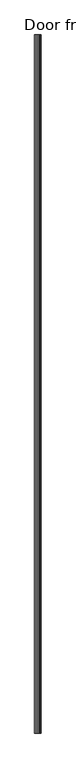
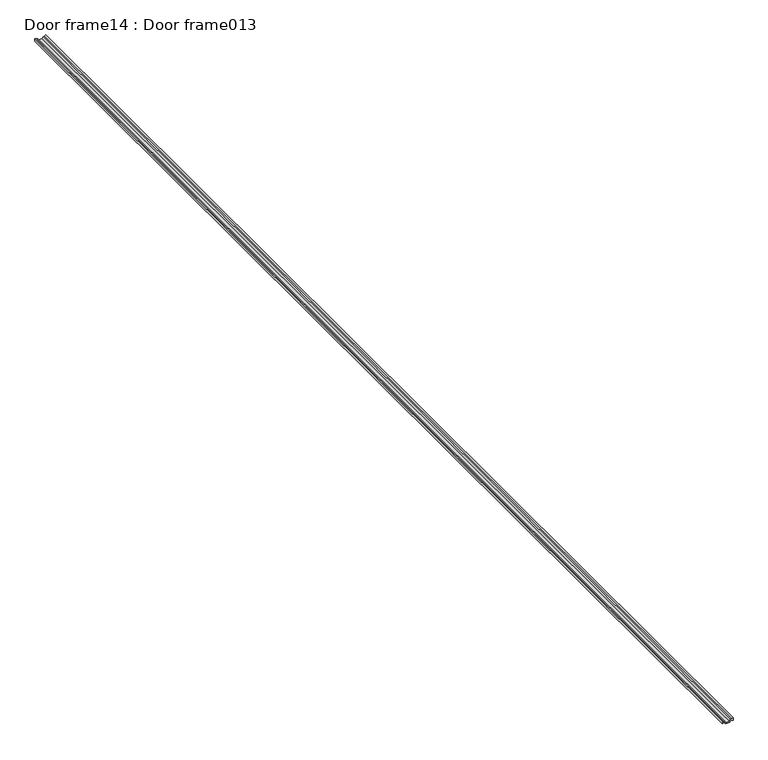
"""IFC4 building model written with IfcOpenShell, lengths in millimetres: proxy geometry, Door frame14 : Door frame013."""

from ifc_helpers import new_model, si_unit, frame, origin, place, context, project, spatial, polyline, outline, extrude, source, transform, mapped, element, save


def door_frame14_door_frame013_088115ce(model_context):
    return source(origin(), model_context, "Body", "SweptSolid", [
        extrude(outline(polyline([(36596.1835829, 15554.7629668), (36596.1835829, 15556.3015659), (36595.1059519, 15558.7219647), (36599.8429954, 15558.7219647), (36598.3174519, 15556.0796459), (36598.3174519, 15554.3038786), (36595.2518099, 15552.157293), (36595.2518099, 15546.8085492), (36598.3174519, 15544.6619636), (36598.3174519, 15542.8861964), (36599.8429954, 15540.2438775), (36595.1059519, 15540.2438775), (36596.1835829, 15542.6642763), (36596.1835829, 15544.2028754), (36593.6518099, 15545.975642), (36593.6518099, 15552.9902003), (36596.1835829, 15554.7629668)])), frame((0.0, -1052.8906567, 0.0), z_axis=(0.0, 1.0, 0.0), x_axis=(0.0, 0.0, 1.0)), (0.0, 0.0, 1.0), 1999.85),
    ])


if __name__ == "__main__":
    model = new_model("IFC4")
    model_context = context("Model", 3, world=origin())
    ifc_project = project(units=[si_unit("LENGTHUNIT", "METRE", prefix="MILLI")], contexts=[model_context])
    site = spatial("IfcSite", under=ifc_project)
    building = spatial("IfcBuilding", under=site)
    placement = place(None, origin())
    door_frame14_door_frame013_shape = door_frame14_door_frame013_088115ce(model_context)
    element("IfcBuildingElementProxy", 1, Name="Door frame14 : Door frame013", ObjectType="Door frame14 : Door frame013", at=placement, inside=building, context=model_context, shape_type="MappedRepresentation", body=[
        mapped(door_frame14_door_frame013_shape, transform((0.0, 0.0, 0.0), x_axis=(1.0, 0.0, 0.0), y_axis=(0.0, 1.0, 0.0), z_axis=(0.0, 0.0, 1.0))),
    ])
    save(model, "model.ifc")

# Revit data of these elements
# Type "Door frame14 : Door frame013"
#   NameOverride = "Door frame013"
# Element 1 (IfcBuildingElementProxy, "Door frame14 : Door frame013")
#   Materials on its faces: "FLEETWOOD SERIES T-3200 SINGLE SWING DOOR FRAME"
# Materials
#   "FLEETWOOD SERIES T-3200 SINGLE SWING DOOR FRAME": class "Unassigned", colour RGB 128 128 128, transparency 0, Cost = 0
